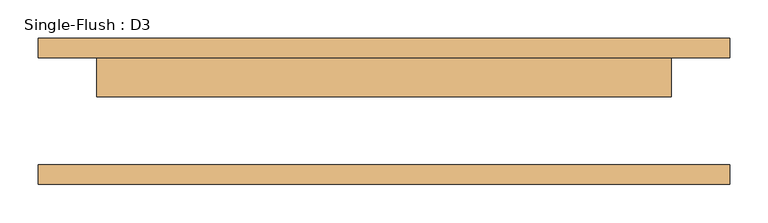
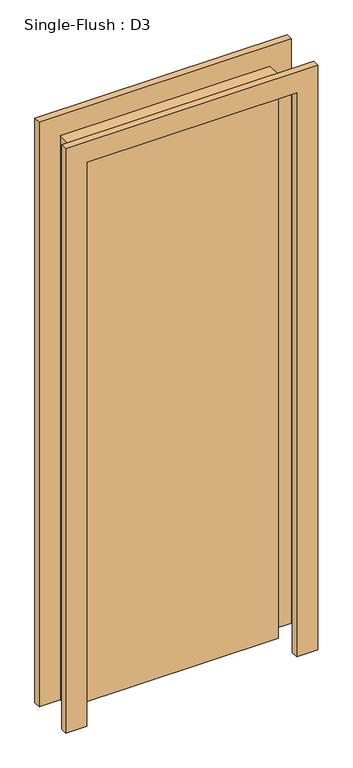
"""IFC4 building model written with IfcOpenShell, lengths in millimetres: door geometry, Single-Flush : D3."""

from ifc_helpers import new_model, si_unit, frame, origin, origin_with_axes, place, context, project, spatial, polyline, outline, extrude, source, transform, mapped, element, save


def single_flush_d3_d87a8d6b(model_context):
    return source(origin(), model_context, "Body", "SweptSolid", [
        extrude(outline(polyline([(2209.8, -451.2), (0.0, -451.2), (0.0, -375.0), (2133.6, -375.0), (2133.6, 375.0), (0.0, 375.0), (0.0, 451.2), (2209.8, 451.2), (2209.8, -451.2)])), frame((0.0, 69.85, 0.0), z_axis=(0.0, 1.0, 0.0), x_axis=(0.0, 0.0, 1.0)), (0.0, 0.0, 1.0), 25.4),
        extrude(outline(polyline([(2209.8, 451.2), (2209.8, -451.2), (0.0, -451.2), (0.0, -375.0), (2133.6, -375.0), (2133.6, 375.0), (0.0, 375.0), (0.0, 451.2), (2209.8, 451.2)])), frame((0.0, -95.25, 0.0), z_axis=(0.0, 1.0, 0.0), x_axis=(0.0, 0.0, 1.0)), (0.0, 0.0, 1.0), 25.4),
        extrude(outline(polyline([(375.0, 19.05), (-375.0, 19.05), (-375.0, 69.85), (375.0, 69.85), (375.0, 19.05)])), origin_with_axes(), (0.0, 0.0, 1.0), 2133.6),
    ])


if __name__ == "__main__":
    model = new_model("IFC4")
    model_context = context("Model", 3, world=origin())
    ifc_project = project(units=[si_unit("LENGTHUNIT", "METRE", prefix="MILLI")], contexts=[model_context])
    site = spatial("IfcSite", under=ifc_project)
    building = spatial("IfcBuilding", under=site)
    placement = place(None, origin())
    single_flush_d3_shape = single_flush_d3_d87a8d6b(model_context)
    element("IfcDoor", 1, ObjectType="Single-Flush : D3", at=placement, inside=building, context=model_context, shape_type="MappedRepresentation", body=[
        mapped(single_flush_d3_shape, transform((0.0, 0.0, 0.0), x_axis=(1.0, 0.0, 0.0), y_axis=(0.0, 1.0, 0.0), z_axis=(0.0, 0.0, 1.0))),
    ])
    save(model, "model.ifc")

# Revit data of these elements
# Type "Single-Flush : D3"
#   Type Mark = "D2"
#   Construction Type Id = "MDOOR"
#   Assembly Code = "C1020"
#   Analytic Construction = "Metal"
#   Thickness = 50.8 mm
#   Heat Transfer Coefficient (U) = 3.7021 W/(m²·K)
#   Height = 2133.6 mm
#   Trim Projection Ext = 25.4 mm
#   Trim Projection Int = 25.4 mm
#   Trim Width = 76.2 mm
#   Width = 750 mm
#   Door Material = Door - Panel
#   Frame Material = Door - Frame
#   Visual Light Transmittance = 0
#   Solar Heat Gain Coefficient = 0
#   Function = (empty or 0)
#   Wall Closure = (empty or 0)
# Element 1 (IfcDoor, "Single-Flush : D3")
#   Materials on its faces: "Door - Frame", "Door - Panel"
# Materials
#   "Door - Panel": class "Wood", colour RGB 210 159 95, transparency 0
#   "Door - Frame": class "Miscellaneous", colour RGB 118 70 51, transparency 0
